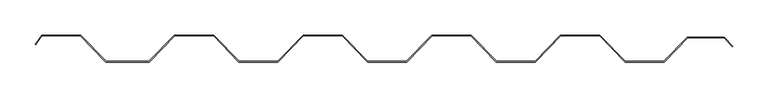
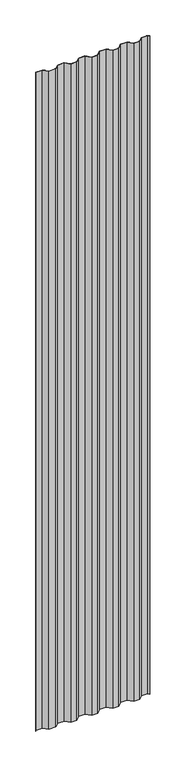
"""IFC4 building model written with IfcOpenShell, lengths in millimetres: proxy geometry, Generic Models 2:Generic Models 2:310765:Generic Models 2:310765 : Generic Models 2:Generic Models 2:310765:2 : Generic Models 2:Generic Models 2:310765:Generic Models 2:310765 : Generic Models 2:Generic Models 2:310765:300385."""

import ifcopenshell
import ifcopenshell.guid

model = None  # the IFC model being written
_history = None  # IfcOwnerHistory: only IFC2X3 demands one
_inside = {}  # id of a spatial element -> (the spatial element, [elements in it])
_under = {}  # id of a project, library or spatial element -> (it, [spatial elements below it])
_declared = {}  # id of a project -> (the project, [libraries it declares])
_typed = {}  # id of a type object -> (the type object, [elements of that type])
_made_of = {}  # id of a material, layer set ... -> (it, [elements and type objects made of it])


def new_model(schema):
    """Start an empty IFC model of exactly this schema.

    Asked for "IFC4X3", IfcOpenShell would pick the latest addendum, in which some entities
    have other attributes; the version numbers below select the first issue.
    IFC2X3 requires an IfcOwnerHistory on every rooted entity: one is made here for all.
    """
    global model, _history
    if schema == "IFC4X3":
        model = ifcopenshell.file(schema_version=(4, 3, 0, 0))
    else:
        model = ifcopenshell.file(schema=schema)
    _inside.clear()
    _under.clear()
    _declared.clear()
    _typed.clear()
    _made_of.clear()
    _history = None
    if model.schema == "IFC2X3":
        org = make("IfcOrganization", Name="unknown")
        user = make(
            "IfcPersonAndOrganization",
            ThePerson=make("IfcPerson", FamilyName="unknown"),
            TheOrganization=org,
        )
        app = make(
            "IfcApplication",
            ApplicationDeveloper=org,
            Version="unknown",
            ApplicationFullName="unknown",
            ApplicationIdentifier="unknown",
        )
        _history = make(
            "IfcOwnerHistory",
            OwningUser=user,
            OwningApplication=app,
            ChangeAction="ADDED",
            CreationDate=0,
        )
    return model


def make(cls, **values):
    """One entity of the class cls with the attributes given. An attribute that is None is left unset."""
    return model.create_entity(
        cls, **{name: value for name, value in values.items() if value is not None}
    )


def rooted(cls, **values):
    """An entity with a GlobalId (a new one), such as an element, a storey or a relation."""
    return make(cls, GlobalId=ifcopenshell.guid.new(), OwnerHistory=_history, **values)


def si_unit(unit_type, name, prefix=None):
    """IfcSIUnit, for example si_unit("LENGTHUNIT", "METRE", prefix="MILLI")."""
    return make("IfcSIUnit", UnitType=unit_type, Prefix=prefix, Name=name)


def assignment(units):
    """IfcUnitAssignment: the units of a project."""
    return None if units is None else make("IfcUnitAssignment", Units=units)


def point(xyz):
    """IfcCartesianPoint."""
    return None if xyz is None else make("IfcCartesianPoint", Coordinates=xyz)


def direction(xyz):
    """IfcDirection."""
    return None if xyz is None else make("IfcDirection", DirectionRatios=xyz)


def frame(location, z_axis=None, x_axis=None):
    """IfcAxis2Placement3D, a coordinate frame: its origin and axes. An axis left out is left unset."""
    return make(
        "IfcAxis2Placement3D",
        Location=point(location),
        Axis=direction(z_axis),
        RefDirection=direction(x_axis),
    )


def origin():
    """The frame at (0, 0, 0) with its axes left unset."""
    return frame((0.0, 0.0, 0.0))


def place(relative_to, where):
    """IfcLocalPlacement: puts the frame where relative to a parent placement (None: the world)."""
    return make(
        "IfcLocalPlacement", PlacementRelTo=relative_to, RelativePlacement=where
    )


def context(
    kind, dimensions, precision=None, world=None, true_north=None, identifier=None
):
    """IfcGeometricRepresentationContext, for example the 3D "Model" context."""
    return make(
        "IfcGeometricRepresentationContext",
        ContextIdentifier=identifier,
        ContextType=kind,
        CoordinateSpaceDimension=dimensions,
        Precision=precision,
        WorldCoordinateSystem=world,
        TrueNorth=true_north,
    )


def project(units=None, contexts=None):
    """IfcProject with its units and contexts."""
    return rooted(
        "IfcProject",
        Name="project",
        RepresentationContexts=contexts,
        UnitsInContext=assignment(units),
    )


def spatial(cls, under=None, at=None, **own):
    """A site, building, storey or space (cls), placed at a placement, below another one or the project."""
    s = rooted(cls, ObjectPlacement=at, **own)
    if under is not None:
        _under.setdefault(under.id(), (under, []))[1].append(s)
    return s


def polyline(points):
    """IfcPolyline through the points."""
    return make("IfcPolyline", Points=[point(p) for p in points])


def outline(outer, holes=None, kind="AREA"):
    """IfcArbitraryClosedProfileDef: a profile drawn as a closed curve; with holes, ...WithVoids."""
    if holes is None:
        return make("IfcArbitraryClosedProfileDef", ProfileType=kind, OuterCurve=outer)
    return make(
        "IfcArbitraryProfileDefWithVoids",
        ProfileType=kind,
        OuterCurve=outer,
        InnerCurves=holes,
    )


def extrude(swept, where, along, depth):
    """IfcExtrudedAreaSolid: the profile swept, set in the frame where, extruded along a direction by depth."""
    return make(
        "IfcExtrudedAreaSolid",
        SweptArea=swept,
        Position=where,
        ExtrudedDirection=direction(along),
        Depth=depth,
    )


def shape(context_of_items, identifier, shape_type, items):
    """IfcShapeRepresentation: the items that make up one representation, for example the "Body"."""
    return make(
        "IfcShapeRepresentation",
        ContextOfItems=context_of_items,
        RepresentationIdentifier=identifier,
        RepresentationType=shape_type,
        Items=items,
    )


def source(mapping_origin, context_of_items, identifier, shape_type, items):
    """IfcRepresentationMap: a shape defined once, which mapped items show again and again."""
    return make(
        "IfcRepresentationMap",
        MappingOrigin=mapping_origin,
        MappedRepresentation=shape(context_of_items, identifier, shape_type, items),
    )


def transform(
    local_origin,
    x_axis=None,
    y_axis=None,
    z_axis=None,
    scale=None,
    scale2=None,
    scale3=None,
    uniform=True,
):
    """IfcCartesianTransformationOperator3D, or its non-uniform kind. x_axis, y_axis, z_axis: its Axis1, 2, 3."""
    if uniform:
        return make(
            "IfcCartesianTransformationOperator3D",
            Axis1=direction(x_axis),
            Axis2=direction(y_axis),
            LocalOrigin=point(local_origin),
            Scale=scale,
            Axis3=direction(z_axis),
        )
    return make(
        "IfcCartesianTransformationOperator3DnonUniform",
        Axis1=direction(x_axis),
        Axis2=direction(y_axis),
        LocalOrigin=point(local_origin),
        Scale=scale,
        Axis3=direction(z_axis),
        Scale2=scale2,
        Scale3=scale3,
    )


def mapped(mapping_source, mapping_target):
    """IfcMappedItem: shows the shape of a source again, moved by a transform."""
    return make(
        "IfcMappedItem", MappingSource=mapping_source, MappingTarget=mapping_target
    )


def made_of(thing, what):
    """Note that an element or type object is made of a material, layer set ...; save() writes the relation."""
    if what is not None:
        _made_of.setdefault(what.id(), (what, []))[1].append(thing)
    return thing


def element(
    cls,
    number,
    at=None,
    inside=None,
    cuts=None,
    type_object=None,
    material=None,
    context=None,
    identifier="Body",
    shape_type=None,
    held_by="IfcProductDefinitionShape",
    body=None,
    shapes=None,
    **own,
):
    """One element of the class cls, such as IfcWall. Its Tag is "e" and its number.

    at: its placement. inside: the storey or other place that contains it. cuts: it is an
    opening in that element (IfcRelVoidsElement). A single representation is given by context,
    identifier, shape_type and body (its items); several are given by shapes. held_by: the class
    of the entity that holds the representations. save() writes the other relations.
    """
    e = rooted(cls, Tag="e%d" % number, ObjectPlacement=at, **own)
    if body is not None:
        shapes = [shape(context, identifier, shape_type, body)]
    if shapes is not None:
        e.Representation = make(held_by, Representations=shapes)
    if inside is not None:
        _inside.setdefault(inside.id(), (inside, []))[1].append(e)
    if cuts is not None:
        rooted(
            "IfcRelVoidsElement", RelatingBuildingElement=cuts, RelatedOpeningElement=e
        )
    if type_object is not None:
        _typed.setdefault(type_object.id(), (type_object, []))[1].append(e)
    return made_of(e, material)


def aggregate(whole, parts):
    """IfcRelAggregates: a whole, such as a stair, and the parts it consists of."""
    return rooted("IfcRelAggregates", RelatingObject=whole, RelatedObjects=parts)


def save(model, path):
    """Write the relations noted so far, then the file.

    IfcRelAggregates (storeys below a building ...), IfcRelContainedInSpatialStructure (elements
    in a storey), IfcRelDefinesByType, IfcRelAssociatesMaterial and IfcRelDeclares: one each for
    every whole, place, type object, material and project.
    """
    for whole, parts in _under.values():
        aggregate(whole, parts)
    for where, things in _inside.values():
        rooted(
            "IfcRelContainedInSpatialStructure",
            RelatedElements=things,
            RelatingStructure=where,
        )
    for kind, things in _typed.values():
        rooted("IfcRelDefinesByType", RelatedObjects=things, RelatingType=kind)
    for what, things in _made_of.values():
        rooted("IfcRelAssociatesMaterial", RelatedObjects=things, RelatingMaterial=what)
    for by, libraries in _declared.values():
        rooted("IfcRelDeclares", RelatingContext=by, RelatedDefinitions=libraries)
    model.write(path)


def generic_models_22e34f16(model_context):
    return source(origin(), model_context, "Body", "SweptSolid", [
        extrude(outline(polyline([(593719.8809779, -536496.5394986), (593731.7367242, -536509.6475696), (593731.1747524, -536510.2095414), (593719.5286406, -536497.3332486), (593667.6222866, -536497.3332486), (593633.9903018, -536531.8913358), (593578.8107419, -536531.8913358), (593542.6485503, -536494.5850858), (593487.2734246, -536494.5850858), (593451.111233, -536531.8913358), (593395.9307419, -536531.8913358), (593359.7685503, -536494.5850858), (593304.3934246, -536494.5850858), (593268.231233, -536531.8913358), (593213.0507419, -536531.8913358), (593176.8885503, -536494.5850858), (593121.5134246, -536494.5850858), (593085.351233, -536531.8913358), (593030.1707419, -536531.8913358), (592994.0085503, -536494.5850858), (592938.6334246, -536494.5850858), (592902.471233, -536531.8913358), (592840.9407419, -536531.8913358), (592804.7785503, -536494.5850858), (592750.2499875, -536494.5850858), (592741.3086193, -536507.3546831), (592740.6584173, -536506.8994068), (592749.8367875, -536493.7913358), (592805.1145958, -536493.7913358), (592841.2767875, -536531.0975858), (592902.1351875, -536531.0975858), (592938.2973791, -536493.7913358), (592994.3445958, -536493.7913358), (593030.5067875, -536531.0975858), (593085.0151875, -536531.0975858), (593121.1773791, -536493.7913358), (593177.2245958, -536493.7913358), (593213.3867875, -536531.0975858), (593267.8951875, -536531.0975858), (593304.0573791, -536493.7913358), (593360.1045958, -536493.7913358), (593396.2667875, -536531.0975858), (593450.7751875, -536531.0975858), (593486.9373791, -536493.7913358), (593542.9845958, -536493.7913358), (593579.1467875, -536531.0975858), (593633.6551875, -536531.0975858), (593667.2871722, -536496.5394986), (593719.8809779, -536496.5394986)])), frame((0.0, 0.0, 2495.55), z_axis=(0.0, 0.0, 1.0), x_axis=(1.0, 0.0, 0.0)), (0.0, 0.0, 1.0), 6069.2190068),
    ])


if __name__ == "__main__":
    model = new_model("IFC4")
    model_context = context("Model", 3, world=origin())
    ifc_project = project(units=[si_unit("LENGTHUNIT", "METRE", prefix="MILLI")], contexts=[model_context])
    site = spatial("IfcSite", under=ifc_project)
    building = spatial("IfcBuilding", under=site)
    placement = place(None, origin())
    generic_models_shape = generic_models_22e34f16(model_context)
    element("IfcBuildingElementProxy", 1, Name="Generic Models 2:Generic Models 2:310765:Generic Models 2:310765 : Generic Models 2:Generic Models 2:310765:2 : Generic Models 2:Generic Models 2:310765:Generic Models 2:310765 : Generic Models 2:Generic Models 2:310765:300385", ObjectType="Generic Models 2:Generic Models 2:310765:Generic Models 2:310765 : Generic Models 2:Generic Models 2:310765:2 : Generic Models 2:Generic Models 2:310765:Generic Models 2:310765 : Generic Models 2:Generic Models 2:310765:300385", at=placement, inside=building, context=model_context, shape_type="MappedRepresentation", body=[
        mapped(generic_models_shape, transform((0.0, 0.0, 0.0), x_axis=(1.0, 0.0, 0.0), y_axis=(0.0, 1.0, 0.0), z_axis=(0.0, 0.0, 1.0))),
    ])
    save(model, "model.ifc")

# Revit data of these elements
# Type "Generic Models 2:Generic Models 2:310765:Generic Models 2:310765 : Generic Models 2:Generic Models 2:310765:2 : Generic Models 2:Generic Models 2:310765:Generic Models 2:310765 : Generic Models 2:Generic Models 2:310765:300385"
#   NameOverride = "Generic Models 2:Generic Models 2:310765:Generic Models 2:310765 : Generic Models 2:Generic Models 2:310765:300385"
#   ObjectTypeOverride = "Generic Models 2:310765 : Generic Models 2:Generic Models 2:310765"
#   Reference = "Generic Models 2"
#   Tag = "300385"
# Element 1 (IfcBuildingElementProxy, "Generic Models 2:Generic Models 2:310765:Generic Models 2:310765 : Generic Models 2:Generic Models 2:310765:2 : Generic Models 2:Generic Models 2:310765:Generic Models 2:310765 : Generic Models 2:Generic Models 2:310765:300385")
#   Materials on its faces: "VERTICAL CORRUGATED METAL PANEL - EXPOSED FASTENERS - (MBCI 7.2 PANEL)"
# Materials
#   "VERTICAL CORRUGATED METAL PANEL - EXPOSED FASTENERS - (MBCI 7.2 PANEL)": class "Generic", colour RGB 120 120 120, transparency 0, Cost = 0
